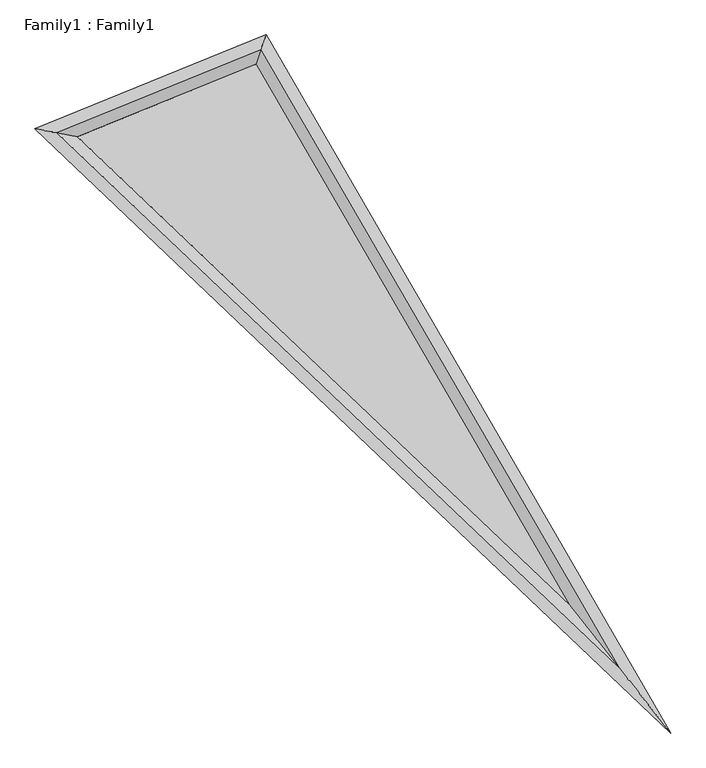
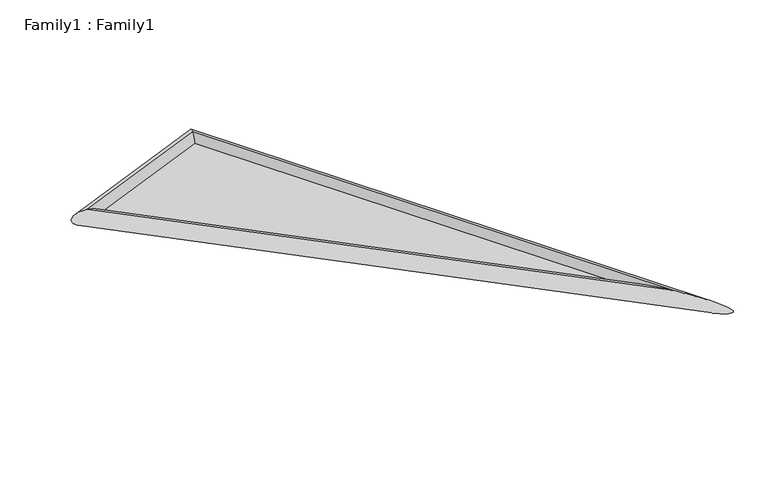
"""IFC4 building model written with IfcOpenShell, lengths in millimetres: proxy geometry, Family1 : Family1."""

import ifcopenshell
import ifcopenshell.guid

model = None  # the IFC model being written
_history = None  # IfcOwnerHistory: only IFC2X3 demands one
_inside = {}  # id of a spatial element -> (the spatial element, [elements in it])
_under = {}  # id of a project, library or spatial element -> (it, [spatial elements below it])
_declared = {}  # id of a project -> (the project, [libraries it declares])
_typed = {}  # id of a type object -> (the type object, [elements of that type])
_made_of = {}  # id of a material, layer set ... -> (it, [elements and type objects made of it])


def new_model(schema):
    """Start an empty IFC model of exactly this schema.

    Asked for "IFC4X3", IfcOpenShell would pick the latest addendum, in which some entities
    have other attributes; the version numbers below select the first issue.
    IFC2X3 requires an IfcOwnerHistory on every rooted entity: one is made here for all.
    """
    global model, _history
    if schema == "IFC4X3":
        model = ifcopenshell.file(schema_version=(4, 3, 0, 0))
    else:
        model = ifcopenshell.file(schema=schema)
    _inside.clear()
    _under.clear()
    _declared.clear()
    _typed.clear()
    _made_of.clear()
    _history = None
    if model.schema == "IFC2X3":
        org = make("IfcOrganization", Name="unknown")
        user = make(
            "IfcPersonAndOrganization",
            ThePerson=make("IfcPerson", FamilyName="unknown"),
            TheOrganization=org,
        )
        app = make(
            "IfcApplication",
            ApplicationDeveloper=org,
            Version="unknown",
            ApplicationFullName="unknown",
            ApplicationIdentifier="unknown",
        )
        _history = make(
            "IfcOwnerHistory",
            OwningUser=user,
            OwningApplication=app,
            ChangeAction="ADDED",
            CreationDate=0,
        )
    return model


def make(cls, **values):
    """One entity of the class cls with the attributes given. An attribute that is None is left unset."""
    return model.create_entity(
        cls, **{name: value for name, value in values.items() if value is not None}
    )


def rooted(cls, **values):
    """An entity with a GlobalId (a new one), such as an element, a storey or a relation."""
    return make(cls, GlobalId=ifcopenshell.guid.new(), OwnerHistory=_history, **values)


def si_unit(unit_type, name, prefix=None):
    """IfcSIUnit, for example si_unit("LENGTHUNIT", "METRE", prefix="MILLI")."""
    return make("IfcSIUnit", UnitType=unit_type, Prefix=prefix, Name=name)


def assignment(units):
    """IfcUnitAssignment: the units of a project."""
    return None if units is None else make("IfcUnitAssignment", Units=units)


def point(xyz):
    """IfcCartesianPoint."""
    return None if xyz is None else make("IfcCartesianPoint", Coordinates=xyz)


def direction(xyz):
    """IfcDirection."""
    return None if xyz is None else make("IfcDirection", DirectionRatios=xyz)


def frame(location, z_axis=None, x_axis=None):
    """IfcAxis2Placement3D, a coordinate frame: its origin and axes. An axis left out is left unset."""
    return make(
        "IfcAxis2Placement3D",
        Location=point(location),
        Axis=direction(z_axis),
        RefDirection=direction(x_axis),
    )


def origin():
    """The frame at (0, 0, 0) with its axes left unset."""
    return frame((0.0, 0.0, 0.0))


def origin_with_axes():
    """The frame at (0, 0, 0) with the z axis (0, 0, 1) and the x axis (1, 0, 0) written out."""
    return frame((0.0, 0.0, 0.0), z_axis=(0.0, 0.0, 1.0), x_axis=(1.0, 0.0, 0.0))


def place(relative_to, where):
    """IfcLocalPlacement: puts the frame where relative to a parent placement (None: the world)."""
    return make(
        "IfcLocalPlacement", PlacementRelTo=relative_to, RelativePlacement=where
    )


def context(
    kind, dimensions, precision=None, world=None, true_north=None, identifier=None
):
    """IfcGeometricRepresentationContext, for example the 3D "Model" context."""
    return make(
        "IfcGeometricRepresentationContext",
        ContextIdentifier=identifier,
        ContextType=kind,
        CoordinateSpaceDimension=dimensions,
        Precision=precision,
        WorldCoordinateSystem=world,
        TrueNorth=true_north,
    )


def project(units=None, contexts=None):
    """IfcProject with its units and contexts."""
    return rooted(
        "IfcProject",
        Name="project",
        RepresentationContexts=contexts,
        UnitsInContext=assignment(units),
    )


def spatial(cls, under=None, at=None, **own):
    """A site, building, storey or space (cls), placed at a placement, below another one or the project."""
    s = rooted(cls, ObjectPlacement=at, **own)
    if under is not None:
        _under.setdefault(under.id(), (under, []))[1].append(s)
    return s


def polyline(points):
    """IfcPolyline through the points."""
    return make("IfcPolyline", Points=[point(p) for p in points])


def ellipse_curve(where, semi_axis1, semi_axis2):
    """IfcEllipse in the frame where."""
    return make(
        "IfcEllipse", Position=where, SemiAxis1=semi_axis1, SemiAxis2=semi_axis2
    )


def outline(outer, holes=None, kind="AREA"):
    """IfcArbitraryClosedProfileDef: a profile drawn as a closed curve; with holes, ...WithVoids."""
    if holes is None:
        return make("IfcArbitraryClosedProfileDef", ProfileType=kind, OuterCurve=outer)
    return make(
        "IfcArbitraryProfileDefWithVoids",
        ProfileType=kind,
        OuterCurve=outer,
        InnerCurves=holes,
    )


def extrude(swept, where, along, depth):
    """IfcExtrudedAreaSolid: the profile swept, set in the frame where, extruded along a direction by depth."""
    return make(
        "IfcExtrudedAreaSolid",
        SweptArea=swept,
        Position=where,
        ExtrudedDirection=direction(along),
        Depth=depth,
    )


def shape(context_of_items, identifier, shape_type, items):
    """IfcShapeRepresentation: the items that make up one representation, for example the "Body"."""
    return make(
        "IfcShapeRepresentation",
        ContextOfItems=context_of_items,
        RepresentationIdentifier=identifier,
        RepresentationType=shape_type,
        Items=items,
    )


def source(mapping_origin, context_of_items, identifier, shape_type, items):
    """IfcRepresentationMap: a shape defined once, which mapped items show again and again."""
    return make(
        "IfcRepresentationMap",
        MappingOrigin=mapping_origin,
        MappedRepresentation=shape(context_of_items, identifier, shape_type, items),
    )


def transform(
    local_origin,
    x_axis=None,
    y_axis=None,
    z_axis=None,
    scale=None,
    scale2=None,
    scale3=None,
    uniform=True,
):
    """IfcCartesianTransformationOperator3D, or its non-uniform kind. x_axis, y_axis, z_axis: its Axis1, 2, 3."""
    if uniform:
        return make(
            "IfcCartesianTransformationOperator3D",
            Axis1=direction(x_axis),
            Axis2=direction(y_axis),
            LocalOrigin=point(local_origin),
            Scale=scale,
            Axis3=direction(z_axis),
        )
    return make(
        "IfcCartesianTransformationOperator3DnonUniform",
        Axis1=direction(x_axis),
        Axis2=direction(y_axis),
        LocalOrigin=point(local_origin),
        Scale=scale,
        Axis3=direction(z_axis),
        Scale2=scale2,
        Scale3=scale3,
    )


def mapped(mapping_source, mapping_target):
    """IfcMappedItem: shows the shape of a source again, moved by a transform."""
    return make(
        "IfcMappedItem", MappingSource=mapping_source, MappingTarget=mapping_target
    )


def made_of(thing, what):
    """Note that an element or type object is made of a material, layer set ...; save() writes the relation."""
    if what is not None:
        _made_of.setdefault(what.id(), (what, []))[1].append(thing)
    return thing


def element(
    cls,
    number,
    at=None,
    inside=None,
    cuts=None,
    type_object=None,
    material=None,
    context=None,
    identifier="Body",
    shape_type=None,
    held_by="IfcProductDefinitionShape",
    body=None,
    shapes=None,
    **own,
):
    """One element of the class cls, such as IfcWall. Its Tag is "e" and its number.

    at: its placement. inside: the storey or other place that contains it. cuts: it is an
    opening in that element (IfcRelVoidsElement). A single representation is given by context,
    identifier, shape_type and body (its items); several are given by shapes. held_by: the class
    of the entity that holds the representations. save() writes the other relations.
    """
    e = rooted(cls, Tag="e%d" % number, ObjectPlacement=at, **own)
    if body is not None:
        shapes = [shape(context, identifier, shape_type, body)]
    if shapes is not None:
        e.Representation = make(held_by, Representations=shapes)
    if inside is not None:
        _inside.setdefault(inside.id(), (inside, []))[1].append(e)
    if cuts is not None:
        rooted(
            "IfcRelVoidsElement", RelatingBuildingElement=cuts, RelatedOpeningElement=e
        )
    if type_object is not None:
        _typed.setdefault(type_object.id(), (type_object, []))[1].append(e)
    return made_of(e, material)


def aggregate(whole, parts):
    """IfcRelAggregates: a whole, such as a stair, and the parts it consists of."""
    return rooted("IfcRelAggregates", RelatingObject=whole, RelatedObjects=parts)


def save(model, path):
    """Write the relations noted so far, then the file.

    IfcRelAggregates (storeys below a building ...), IfcRelContainedInSpatialStructure (elements
    in a storey), IfcRelDefinesByType, IfcRelAssociatesMaterial and IfcRelDeclares: one each for
    every whole, place, type object, material and project.
    """
    for whole, parts in _under.values():
        aggregate(whole, parts)
    for where, things in _inside.values():
        rooted(
            "IfcRelContainedInSpatialStructure",
            RelatedElements=things,
            RelatingStructure=where,
        )
    for kind, things in _typed.values():
        rooted("IfcRelDefinesByType", RelatedObjects=things, RelatingType=kind)
    for what, things in _made_of.values():
        rooted("IfcRelAssociatesMaterial", RelatedObjects=things, RelatingMaterial=what)
    for by, libraries in _declared.values():
        rooted("IfcRelDeclares", RelatingContext=by, RelatedDefinitions=libraries)
    model.write(path)


def cylinder_surface(at, radius):
    """IfcCylindricalSurface: all points at the distance radius from the z axis of the frame at."""
    return make("IfcCylindricalSurface", Position=at, Radius=radius)


def advanced_brep(points, edges, surfaces, faces):
    """IfcAdvancedBrep: a solid bounded by faces that lie on surfaces and meet in shared edges.

    An edge is (start, end): straight between two places in points (the first is 0);
    or (start, end, curve); or (start, end, curve, False) where it runs against its curve.
    A face is (place in surfaces, loops), or (place, loops, False) where it looks against
    its surface's normal. A loop lists edges by number (the first is 1), with a minus sign
    where the edge is run from its end to its start. The first loop is the outer one.
    """
    corners = [point(p) for p in points]
    vertices = [make("IfcVertexPoint", VertexGeometry=c) for c in corners]
    made = []
    for start, end, *more in edges:
        made.append(
            make(
                "IfcEdgeCurve",
                EdgeStart=vertices[start],
                EdgeEnd=vertices[end],
                EdgeGeometry=more[0] if more else make("IfcPolyline", Points=[corners[start], corners[end]]),
                SameSense=more[1] if len(more) > 1 else True,
            )
        )
    hull = []
    for where, loops, *sense in faces:
        bounds = []
        for j, loop in enumerate(loops):
            ring = [make("IfcOrientedEdge", EdgeElement=made[abs(k) - 1], Orientation=k > 0) for k in loop]
            bounds.append(
                make(
                    "IfcFaceOuterBound" if j == 0 else "IfcFaceBound",
                    Bound=make("IfcEdgeLoop", EdgeList=ring),
                    Orientation=True,
                )
            )
        hull.append(make("IfcAdvancedFace", Bounds=bounds, FaceSurface=surfaces[where], SameSense=sense[0] if sense else True))
    return make("IfcAdvancedBrep", Outer=make("IfcClosedShell", CfsFaces=hull))


def family1_family1_f69f1062(model_context):
    return source(origin(), model_context, "Body", "SolidModel", [
        extrude(outline(polyline([(3477.0900612, -2737.1084537), (-1206.1623048, 1715.1759376), (495.9946945, 2405.873721), (3477.0900612, -2737.1084537)])), origin_with_axes(), (0.0, 0.0, 1.0), 34.1328789),
        advanced_brep(
        [(3477.0900612, -2737.1084537, 100.0), (3477.0900612, -2737.1084537, -100.0), (-1206.1623048, 1715.1759376, -100.0), (-1206.1623048, 1715.1759376, 100.0), (495.9946945, 2405.873721, -100.0), (495.9946945, 2405.873721, 100.0)],
        [
            (0, 1, ellipse_curve(frame((3477.0900612, -2737.1084537, 0.0), z_axis=(-0.7850645424277253, -0.6194139683787785, 0.0), x_axis=(0.6194139683787784, -0.7850645424277254, 0.0)), 703.2569664, 100.0)),
            (1, 2),
            (2, 3, ellipse_curve(frame((-1206.1623048, 1715.1759376, 0.0), z_axis=(-0.18622829424799262, -0.9825064999385414, 0.0), x_axis=(0.9825064999385414, -0.18622829424799253, 0.0)), 184.5063833, 100.0)),
            (3, 0),
            (1, 0, ellipse_curve(frame((3477.0900612, -2737.1084537, 0.0), z_axis=(-0.7850645424277253, -0.6194139683787785, 0.0), x_axis=(0.6194139683787784, -0.7850645424277254, 0.0)), 703.2569664, 100.0)),
            (3, 2, ellipse_curve(frame((-1206.1623048, 1715.1759376, 0.0), z_axis=(-0.18622829424799262, -0.9825064999385414, 0.0), x_axis=(0.9825064999385414, -0.18622829424799253, 0.0)), 184.5063833, 100.0)),
            (2, 4),
            (4, 5, ellipse_curve(frame((495.9946945, 2405.873721, 0.0), z_axis=(-0.9460420147060632, 0.32404398838875764, 0.0), x_axis=(-0.32404398838875714, -0.9460420147060632, 0.0)), 132.4890283, 100.0)),
            (5, 3),
            (5, 4, ellipse_curve(frame((495.9946945, 2405.873721, 0.0), z_axis=(-0.9460420147060632, 0.32404398838875764, 0.0), x_axis=(-0.32404398838875714, -0.9460420147060632, 0.0)), 132.4890283, 100.0)),
            (4, 1),
            (0, 5),
        ],
        [
            cylinder_surface(frame((3477.0900612, -2737.1084537, 0.0), z_axis=(0.7247525197450744, -0.6890092779659543, 0.0), x_axis=(-0.6890092779659543, -0.7247525197450744, 0.0)), 100.0),
            cylinder_surface(frame((-1206.1623048, 1715.1759376, 0.0), z_axis=(-0.9266190253478895, -0.37600157162348036, 0.0), x_axis=(-0.37600157162348036, 0.9266190253478895, 0.0)), 100.0),
            cylinder_surface(frame((495.9946945, 2405.873721, 0.0), z_axis=(-0.5014871758045593, 0.8651650781807869, 0.0), x_axis=(0.8651650781807869, 0.5014871758045593, 0.0)), 100.0),
        ],
        [
            (0, [[1, 2, 3, 4]]),
            (0, [[5, -4, 6, -2]]),
            (1, [[-3, 7, 8, 9]]),
            (1, [[-6, -9, 10, -7]]),
            (2, [[-8, 11, -1, 12]]),
            (2, [[-10, -12, -5, -11]]),
        ],
    ),
    ])


if __name__ == "__main__":
    model = new_model("IFC4")
    model_context = context("Model", 3, world=origin())
    ifc_project = project(units=[si_unit("LENGTHUNIT", "METRE", prefix="MILLI")], contexts=[model_context])
    site = spatial("IfcSite", under=ifc_project)
    building = spatial("IfcBuilding", under=site)
    placement = place(None, origin())
    family1_family1_shape = family1_family1_f69f1062(model_context)
    element("IfcBuildingElementProxy", 1, Name="Family1 : Family1", ObjectType="Family1 : Family1", at=placement, inside=building, context=model_context, shape_type="MappedRepresentation", body=[
        mapped(family1_family1_shape, transform((0.0, 0.0, 0.0), x_axis=(1.0, 0.0, 0.0), y_axis=(0.0, 1.0, 0.0), z_axis=(0.0, 0.0, 1.0))),
    ])
    save(model, "model.ifc")

# Revit data of these elements
# Type "Family1 : Family1"
#   Default Elevation = 0
# Element 1 (IfcBuildingElementProxy, "Family1 : Family1")
#   Materials on its faces: "Glass"
# Materials
#   "Glass": class "Glass", colour RGB 0 128 192, transparency 0.9, Description = "Soda Lime Glass", Cost = 0
